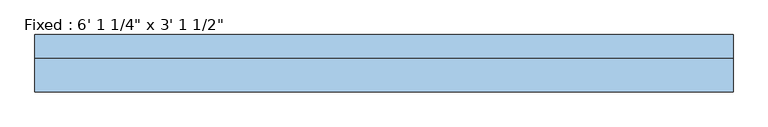
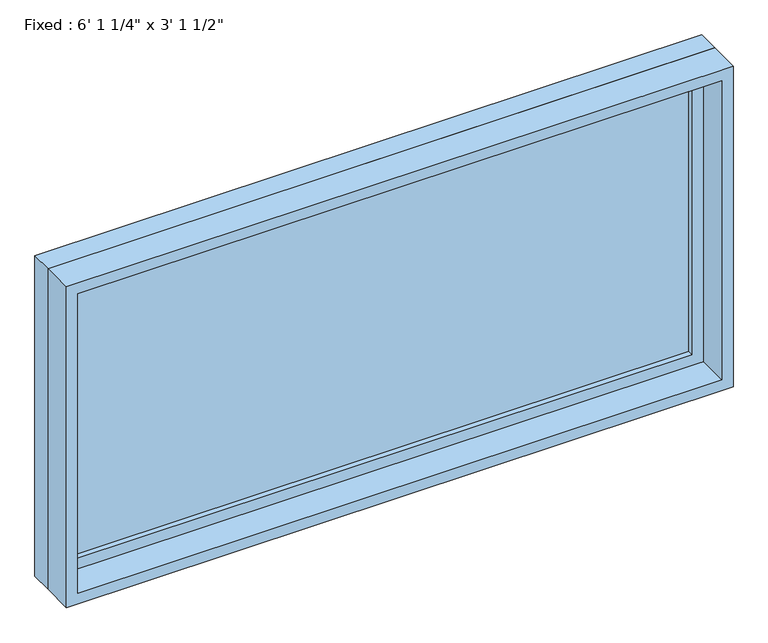
"""IFC4 building model written with IfcOpenShell, lengths in millimetres: window geometry."""

from ifc_helpers import new_model, si_unit, frame, origin, place, context, project, spatial, polyline, outline, extrude, source, transform, mapped, element, save


def window_8dfeb670(model_context):
    return source(origin(), model_context, "Body", "SweptSolid", [
        extrude(outline(polyline([(828.675, 28.575), (-904.875, 28.575), (-904.875, 41.275), (828.675, 41.275), (828.675, 28.575)])), frame((0.0, 0.0, 1257.3), z_axis=(0.0, 0.0, 1.0), x_axis=(1.0, 0.0, 0.0)), (0.0, 0.0, 1.0), 819.15),
        extrude(outline(polyline([(2120.9, -949.325), (1212.85, -949.325), (1212.85, 873.125), (2120.9, 873.125), (2120.9, -949.325)]), holes=[polyline([(2076.45, -904.875), (2076.45, 828.675), (1257.3, 828.675), (1257.3, -904.875), (2076.45, -904.875)])]), frame((0.0, 12.7, 0.0), z_axis=(0.0, 1.0, 0.0), x_axis=(0.0, 0.0, 1.0)), (0.0, 0.0, 1.0), 44.45),
        extrude(outline(polyline([(2139.95, -968.375), (1193.8, -968.375), (1193.8, 892.175), (2139.95, 892.175), (2139.95, -968.375)]), holes=[polyline([(2108.2, -936.625), (2108.2, 860.425), (1225.55, 860.425), (1225.55, -936.625), (2108.2, -936.625)])]), frame((0.0, -76.2, 0.0), z_axis=(0.0, 1.0, 0.0), x_axis=(0.0, 0.0, 1.0)), (0.0, 0.0, 1.0), 88.9),
        extrude(outline(polyline([(2139.95, 892.175), (2139.95, -968.375), (1193.8, -968.375), (1193.8, 892.175), (2139.95, 892.175)]), holes=[polyline([(2120.9, 873.125), (1212.85, 873.125), (1212.85, -949.325), (2120.9, -949.325), (2120.9, 873.125)])]), frame((0.0, 12.7, 0.0), z_axis=(0.0, 1.0, 0.0), x_axis=(0.0, 0.0, 1.0)), (0.0, 0.0, 1.0), 63.5),
    ])


if __name__ == "__main__":
    model = new_model("IFC4")
    model_context = context("Model", 3, world=origin())
    ifc_project = project(units=[si_unit("LENGTHUNIT", "METRE", prefix="MILLI")], contexts=[model_context])
    site = spatial("IfcSite", under=ifc_project)
    building = spatial("IfcBuilding", under=site)
    placement = place(None, origin())
    window_shape = window_8dfeb670(model_context)
    element("IfcWindow", 1, ObjectType="Fixed : 6' 1 1/4\" x 3' 1 1/2\"", at=placement, inside=building, context=model_context, shape_type="MappedRepresentation", body=[
        mapped(window_shape, transform((0.0, 0.0, 0.0), x_axis=(1.0, 0.0, 0.0), y_axis=(0.0, 1.0, 0.0), z_axis=(0.0, 0.0, 1.0))),
    ])
    save(model, "model.ifc")

# Revit data of these elements
# Type "Fixed : 6' 1 1/4\" x 3' 1 1/2\""
#   Type Mark = "21"
#   Assembly Code = "B2020100"
#   Height = 3' - 1 1/4"
#   Default Sill Height = 3' - 11"
#   Width = 6' - 1 1/4"
#   Window Inset = 0' - 0 3/4"
#   Glass Pane Material = Glass
#   Sash Material = Sash
#   Wall Closure = (empty or 0)
# Element 1 (IfcWindow, "Fixed : 6' 1 1/4\" x 3' 1 1/2\"")
#   Materials on its faces: "Sash", "Glass"
# Materials
#   "Glass": class "Glass", colour RGB 218 227 224, transparency 0.85, Description = "Soda Lime Glass", Cost = 0
#   "Sash": class "Wood", colour RGB 136 99 55, transparency 0
